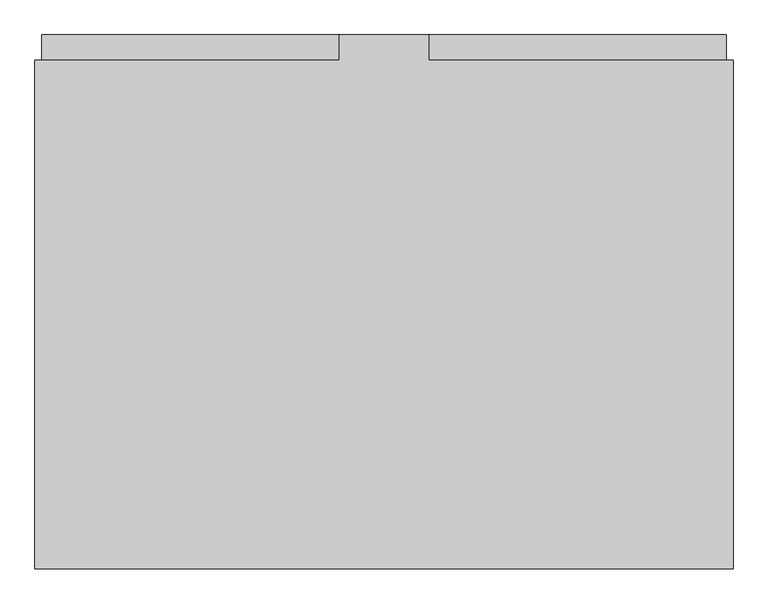
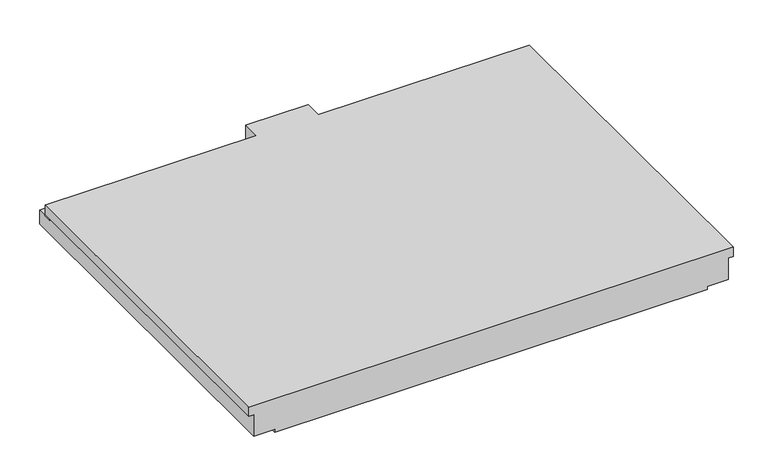
"""IFC4 building model written with IfcOpenShell, lengths in millimetres: stair geometry, NLRS_24_GM_UN_rechthoekig bordes prefab-AV_gen_rsf : prefab bordes_gen__2300x3005."""

import ifcopenshell
import ifcopenshell.guid

model = None  # the IFC model being written
_history = None  # IfcOwnerHistory: only IFC2X3 demands one
_inside = {}  # id of a spatial element -> (the spatial element, [elements in it])
_under = {}  # id of a project, library or spatial element -> (it, [spatial elements below it])
_declared = {}  # id of a project -> (the project, [libraries it declares])
_typed = {}  # id of a type object -> (the type object, [elements of that type])
_made_of = {}  # id of a material, layer set ... -> (it, [elements and type objects made of it])


def new_model(schema):
    """Start an empty IFC model of exactly this schema.

    Asked for "IFC4X3", IfcOpenShell would pick the latest addendum, in which some entities
    have other attributes; the version numbers below select the first issue.
    IFC2X3 requires an IfcOwnerHistory on every rooted entity: one is made here for all.
    """
    global model, _history
    if schema == "IFC4X3":
        model = ifcopenshell.file(schema_version=(4, 3, 0, 0))
    else:
        model = ifcopenshell.file(schema=schema)
    _inside.clear()
    _under.clear()
    _declared.clear()
    _typed.clear()
    _made_of.clear()
    _history = None
    if model.schema == "IFC2X3":
        org = make("IfcOrganization", Name="unknown")
        user = make(
            "IfcPersonAndOrganization",
            ThePerson=make("IfcPerson", FamilyName="unknown"),
            TheOrganization=org,
        )
        app = make(
            "IfcApplication",
            ApplicationDeveloper=org,
            Version="unknown",
            ApplicationFullName="unknown",
            ApplicationIdentifier="unknown",
        )
        _history = make(
            "IfcOwnerHistory",
            OwningUser=user,
            OwningApplication=app,
            ChangeAction="ADDED",
            CreationDate=0,
        )
    return model


def make(cls, **values):
    """One entity of the class cls with the attributes given. An attribute that is None is left unset."""
    return model.create_entity(
        cls, **{name: value for name, value in values.items() if value is not None}
    )


def rooted(cls, **values):
    """An entity with a GlobalId (a new one), such as an element, a storey or a relation."""
    return make(cls, GlobalId=ifcopenshell.guid.new(), OwnerHistory=_history, **values)


def si_unit(unit_type, name, prefix=None):
    """IfcSIUnit, for example si_unit("LENGTHUNIT", "METRE", prefix="MILLI")."""
    return make("IfcSIUnit", UnitType=unit_type, Prefix=prefix, Name=name)


def assignment(units):
    """IfcUnitAssignment: the units of a project."""
    return None if units is None else make("IfcUnitAssignment", Units=units)


def point(xyz):
    """IfcCartesianPoint."""
    return None if xyz is None else make("IfcCartesianPoint", Coordinates=xyz)


def direction(xyz):
    """IfcDirection."""
    return None if xyz is None else make("IfcDirection", DirectionRatios=xyz)


def frame(location, z_axis=None, x_axis=None):
    """IfcAxis2Placement3D, a coordinate frame: its origin and axes. An axis left out is left unset."""
    return make(
        "IfcAxis2Placement3D",
        Location=point(location),
        Axis=direction(z_axis),
        RefDirection=direction(x_axis),
    )


def origin():
    """The frame at (0, 0, 0) with its axes left unset."""
    return frame((0.0, 0.0, 0.0))


def place(relative_to, where):
    """IfcLocalPlacement: puts the frame where relative to a parent placement (None: the world)."""
    return make(
        "IfcLocalPlacement", PlacementRelTo=relative_to, RelativePlacement=where
    )


def context(
    kind, dimensions, precision=None, world=None, true_north=None, identifier=None
):
    """IfcGeometricRepresentationContext, for example the 3D "Model" context."""
    return make(
        "IfcGeometricRepresentationContext",
        ContextIdentifier=identifier,
        ContextType=kind,
        CoordinateSpaceDimension=dimensions,
        Precision=precision,
        WorldCoordinateSystem=world,
        TrueNorth=true_north,
    )


def project(units=None, contexts=None):
    """IfcProject with its units and contexts."""
    return rooted(
        "IfcProject",
        Name="project",
        RepresentationContexts=contexts,
        UnitsInContext=assignment(units),
    )


def spatial(cls, under=None, at=None, **own):
    """A site, building, storey or space (cls), placed at a placement, below another one or the project."""
    s = rooted(cls, ObjectPlacement=at, **own)
    if under is not None:
        _under.setdefault(under.id(), (under, []))[1].append(s)
    return s


def faces_of(points, faces, orient=None, outer=None):
    """IfcFace entities. A face is a list of loops; a loop is a list of indices into points, from 0.

    orient and outer hold one flag for each loop. By default every Orientation is true, the
    first loop of a face is its IfcFaceOuterBound and the others are IfcFaceBound.
    """
    made = []
    for i, loops in enumerate(faces):
        bounds = []
        for j, loop in enumerate(loops):
            is_outer = j == 0 if outer is None else outer[i][j]
            bounds.append(
                make(
                    "IfcFaceOuterBound" if is_outer else "IfcFaceBound",
                    Bound=make("IfcPolyLoop", Polygon=[points[k] for k in loop]),
                    Orientation=True if orient is None else orient[i][j],
                )
            )
        made.append(make("IfcFace", Bounds=bounds))
    return made


def faceted_brep(points, faces, orient=None, outer=None, voids=None):
    """IfcFacetedBrep: a solid bounded by flat faces; with voids (closed shells), ...WithVoids."""
    shared = [point(p) for p in points]
    hull = make("IfcClosedShell", CfsFaces=faces_of(shared, faces, orient, outer))
    if voids is None:
        return make("IfcFacetedBrep", Outer=hull)
    return make(
        "IfcFacetedBrepWithVoids",
        Outer=hull,
        Voids=[
            make(cls, CfsFaces=faces_of(shared, fs, o, b)) for cls, fs, o, b in voids
        ],
    )


def shape(context_of_items, identifier, shape_type, items):
    """IfcShapeRepresentation: the items that make up one representation, for example the "Body"."""
    return make(
        "IfcShapeRepresentation",
        ContextOfItems=context_of_items,
        RepresentationIdentifier=identifier,
        RepresentationType=shape_type,
        Items=items,
    )


def source(mapping_origin, context_of_items, identifier, shape_type, items):
    """IfcRepresentationMap: a shape defined once, which mapped items show again and again."""
    return make(
        "IfcRepresentationMap",
        MappingOrigin=mapping_origin,
        MappedRepresentation=shape(context_of_items, identifier, shape_type, items),
    )


def transform(
    local_origin,
    x_axis=None,
    y_axis=None,
    z_axis=None,
    scale=None,
    scale2=None,
    scale3=None,
    uniform=True,
):
    """IfcCartesianTransformationOperator3D, or its non-uniform kind. x_axis, y_axis, z_axis: its Axis1, 2, 3."""
    if uniform:
        return make(
            "IfcCartesianTransformationOperator3D",
            Axis1=direction(x_axis),
            Axis2=direction(y_axis),
            LocalOrigin=point(local_origin),
            Scale=scale,
            Axis3=direction(z_axis),
        )
    return make(
        "IfcCartesianTransformationOperator3DnonUniform",
        Axis1=direction(x_axis),
        Axis2=direction(y_axis),
        LocalOrigin=point(local_origin),
        Scale=scale,
        Axis3=direction(z_axis),
        Scale2=scale2,
        Scale3=scale3,
    )


def mapped(mapping_source, mapping_target):
    """IfcMappedItem: shows the shape of a source again, moved by a transform."""
    return make(
        "IfcMappedItem", MappingSource=mapping_source, MappingTarget=mapping_target
    )


def made_of(thing, what):
    """Note that an element or type object is made of a material, layer set ...; save() writes the relation."""
    if what is not None:
        _made_of.setdefault(what.id(), (what, []))[1].append(thing)
    return thing


def element(
    cls,
    number,
    at=None,
    inside=None,
    cuts=None,
    type_object=None,
    material=None,
    context=None,
    identifier="Body",
    shape_type=None,
    held_by="IfcProductDefinitionShape",
    body=None,
    shapes=None,
    **own,
):
    """One element of the class cls, such as IfcWall. Its Tag is "e" and its number.

    at: its placement. inside: the storey or other place that contains it. cuts: it is an
    opening in that element (IfcRelVoidsElement). A single representation is given by context,
    identifier, shape_type and body (its items); several are given by shapes. held_by: the class
    of the entity that holds the representations. save() writes the other relations.
    """
    e = rooted(cls, Tag="e%d" % number, ObjectPlacement=at, **own)
    if body is not None:
        shapes = [shape(context, identifier, shape_type, body)]
    if shapes is not None:
        e.Representation = make(held_by, Representations=shapes)
    if inside is not None:
        _inside.setdefault(inside.id(), (inside, []))[1].append(e)
    if cuts is not None:
        rooted(
            "IfcRelVoidsElement", RelatingBuildingElement=cuts, RelatedOpeningElement=e
        )
    if type_object is not None:
        _typed.setdefault(type_object.id(), (type_object, []))[1].append(e)
    return made_of(e, material)


def aggregate(whole, parts):
    """IfcRelAggregates: a whole, such as a stair, and the parts it consists of."""
    return rooted("IfcRelAggregates", RelatingObject=whole, RelatedObjects=parts)


def save(model, path):
    """Write the relations noted so far, then the file.

    IfcRelAggregates (storeys below a building ...), IfcRelContainedInSpatialStructure (elements
    in a storey), IfcRelDefinesByType, IfcRelAssociatesMaterial and IfcRelDeclares: one each for
    every whole, place, type object, material and project.
    """
    for whole, parts in _under.values():
        aggregate(whole, parts)
    for where, things in _inside.values():
        rooted(
            "IfcRelContainedInSpatialStructure",
            RelatedElements=things,
            RelatingStructure=where,
        )
    for kind, things in _typed.values():
        rooted("IfcRelDefinesByType", RelatedObjects=things, RelatingType=kind)
    for what, things in _made_of.values():
        rooted("IfcRelAssociatesMaterial", RelatedObjects=things, RelatingMaterial=what)
    for by, libraries in _declared.values():
        rooted("IfcRelDeclares", RelatingContext=by, RelatedDefinitions=libraries)
    model.write(path)


def stair_f0e5f7b1(model_context):
    return source(origin(), model_context, "Body", "Brep", [
        faceted_brep([(1502.5, 2190.0, 0.0), (1502.5, 0.0, 0.0), (1502.5, 0.0, -60.0), (1502.5, 2190.0, -60.0), (192.5, 2300.0, -110.0), (192.5, 2190.0, -110.0), (1472.5, 2190.0, -110.0), (1472.5, 2300.0, -110.0), (192.5, 2190.0, 0.0), (1472.5, 2190.0, -60.0), (192.5, 2300.0, 0.0), (-192.5, 2300.0, 0.0), (-192.5, 2300.0, -110.0), (-192.5, 2190.0, -110.0), (-192.5, 2190.0, 0.0), (-1502.5, 0.0, 0.0), (-1502.5, 2190.0, 0.0), (-1502.5, 2190.0, -60.0), (-1502.5, 0.0, -60.0), (-1472.5, 2300.0, -110.0), (1472.5, 2300.0, -200.0), (1342.5, 2300.0, -200.0), (1342.5, 2300.0, -220.0), (-1342.5, 2300.0, -220.0), (-1342.5, 2300.0, -200.0), (-1472.5, 2300.0, -200.0), (-1472.5, 2190.0, -110.0), (-1472.5, 2190.0, -60.0), (-1472.5, 0.0, -60.0), (-1472.5, 0.0, -200.0), (-1342.5, 0.0, -200.0), (-1342.5, 0.0, -220.0), (1342.5, 0.0, -220.0), (1342.5, 0.0, -200.0), (1472.5, 0.0, -200.0), (1472.5, 0.0, -60.0)], [[[0, 1, 2, 3]], [[4, 5, 6, 7]], [[8, 0, 3, 9, 6, 5]], [[10, 8, 5, 4]], [[11, 12, 13, 14]], [[15, 16, 17, 18]], [[19, 12, 11, 10, 4, 7, 20, 21, 22, 23, 24, 25]], [[12, 19, 26, 13]], [[16, 14, 13, 26, 27, 17]], [[16, 15, 1, 0, 8, 10, 11, 14]], [[15, 18, 28, 29, 30, 31, 32, 33, 34, 35, 2, 1]], [[31, 23, 22, 32]], [[27, 28, 18, 17]], [[25, 29, 28, 27, 26, 19]], [[29, 25, 24, 30]], [[30, 24, 23, 31]], [[35, 9, 3, 2]], [[34, 20, 7, 6, 9, 35]], [[20, 34, 33, 21]], [[21, 33, 32, 22]]]),
    ])


if __name__ == "__main__":
    model = new_model("IFC4")
    model_context = context("Model", 3, world=origin())
    ifc_project = project(units=[si_unit("LENGTHUNIT", "METRE", prefix="MILLI")], contexts=[model_context])
    site = spatial("IfcSite", under=ifc_project)
    building = spatial("IfcBuilding", under=site)
    placement = place(None, origin())
    stair_shape = stair_f0e5f7b1(model_context)
    element("IfcStair", 1, ObjectType="NLRS_24_GM_UN_rechthoekig bordes prefab-AV_gen_rsf : prefab bordes_gen__2300x3005", at=placement, inside=building, context=model_context, shape_type="MappedRepresentation", body=[
        mapped(stair_shape, transform((0.0, 0.0, 0.0), x_axis=(1.0, 0.0, 0.0), y_axis=(0.0, 1.0, 0.0), z_axis=(0.0, 0.0, 1.0))),
    ])
    save(model, "model.ifc")

# Revit data of these elements
# Type "NLRS_24_GM_UN_rechthoekig bordes prefab-AV_gen_rsf : prefab bordes_gen__2300x3005"
#   IfcExportAs = "IfcStair"
#   Type Comments = " "
#   Model = " "
#   Manufacturer = " "
#   Description = "rechthoekig bordes prefab\r\n1930x4395"
#   Assembly Code = "24.15"
#   Width = 3005 mm
#   Thickness = 220 mm
#   Perimeter = 10610 mm
#   NLRS_C_lengte_02 = 1310 mm
#   NLRS_C_lengte_01 = 1310 mm
#   NLRS_C_hoogte_02 = 110 mm
#   NLRS_C_hoogte_01 = 110 mm
#   NLRS_C_diepte_04 = 2300 mm
#   NLRS_C_diepte_03 = 2300 mm
#   NLRS_C_diepte_02 = 110 mm
#   NLRS_C_diepte_01 = 110 mm
#   Length = 2300 mm
#   Default Elevation = 1219.2 mm
#   Area = 6.9115 m²
#   NLRS_C_materiaal = NLRS_f2_beton prefab_gen_rsf
#   Keynote = ""
# Element 1 (IfcStair, "NLRS_24_GM_UN_rechthoekig bordes prefab-AV_gen_rsf : prefab bordes_gen__2300x3005")
#   Materials on its faces: "NLRS_f2_beton prefab_gen_rsf"
# Materials
#   "NLRS_f2_beton prefab_gen_rsf": class "F - Niet gebakken kunststeen", colour RGB 129 133 118, transparency 0, Keynote = "f2", Manufacturer = "Revit Standards Foundation", URL = "www.revitstandards.org", Description = "beton prefab", Cost = 0
